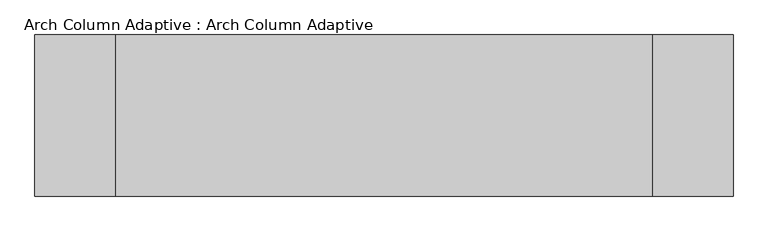
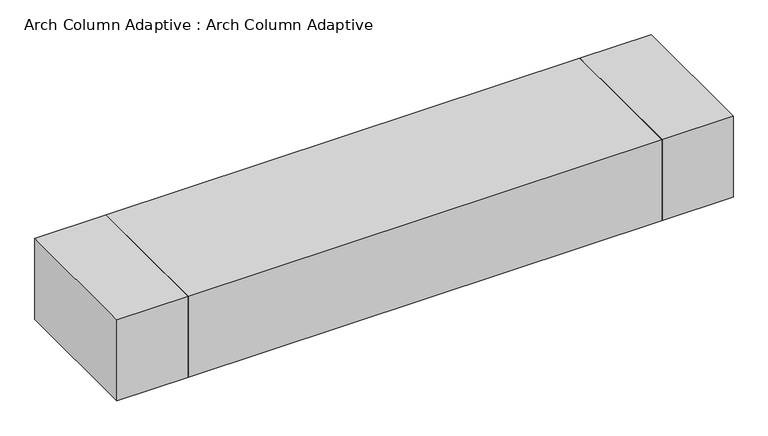
"""IFC4 building model written with IfcOpenShell, lengths in millimetres: proxy geometry, Arch Column Adaptive : Arch Column Adaptive."""

from ifc_helpers import new_model, si_unit, frame, origin, place, context, project, spatial, polyline, outline, extrude, source, transform, mapped, element, save


def arch_column_adaptive_arch_column_adaptive_582f5647(model_context):
    return source(origin(), model_context, "Body", "SweptSolid", [
        extrude(outline(polyline([(5000.0, -1500.0), (5000.0, 1500.0), (6500.0, 1500.0), (6500.0, -1500.0), (5000.0, -1500.0)])), frame((0.0, 0.0, 43700.0), z_axis=(0.0, 0.0, 1.0), x_axis=(1.0, 0.0, 0.0)), (0.0, 0.0, 1.0), 1800.0),
        extrude(outline(polyline([(-5000.0, 1500.0), (-5000.0, -1500.0), (-6500.0, -1500.0), (-6500.0, 1500.0), (-5000.0, 1500.0)])), frame((0.0, 0.0, 43700.0), z_axis=(0.0, 0.0, 1.0), x_axis=(1.0, 0.0, 0.0)), (0.0, 0.0, 1.0), 1800.0),
        extrude(outline(polyline([(-5000.0, -1500.0), (-5000.0, 1500.0), (5000.0, 1500.0), (5000.0, -1500.0), (-5000.0, -1500.0)])), frame((0.0, 0.0, 43700.0), z_axis=(0.0, 0.0, 1.0), x_axis=(1.0, 0.0, 0.0)), (0.0, 0.0, 1.0), 1800.0),
    ])


if __name__ == "__main__":
    model = new_model("IFC4")
    model_context = context("Model", 3, world=origin())
    ifc_project = project(units=[si_unit("LENGTHUNIT", "METRE", prefix="MILLI")], contexts=[model_context])
    site = spatial("IfcSite", under=ifc_project)
    building = spatial("IfcBuilding", under=site)
    placement = place(None, origin())
    arch_column_adaptive_arch_column_adaptive_shape = arch_column_adaptive_arch_column_adaptive_582f5647(model_context)
    element("IfcBuildingElementProxy", 1, Name="Arch Column Adaptive : Arch Column Adaptive", ObjectType="Arch Column Adaptive : Arch Column Adaptive", at=placement, inside=building, context=model_context, shape_type="MappedRepresentation", body=[
        mapped(arch_column_adaptive_arch_column_adaptive_shape, transform((0.0, 0.0, 0.0), x_axis=(1.0, 0.0, 0.0), y_axis=(0.0, 1.0, 0.0), z_axis=(0.0, 0.0, 1.0))),
    ])
    save(model, "model.ifc")

# Revit data of these elements
# Type "Arch Column Adaptive : Arch Column Adaptive"
#   Top Width = 3000 mm
#   Length [instance default] = 21000 mm
#   Height [instance default] = 50000 mm
#   Default Elevation = 0
# Element 1 (IfcBuildingElementProxy, "Arch Column Adaptive : Arch Column Adaptive")
#   Height = 43700 mm
